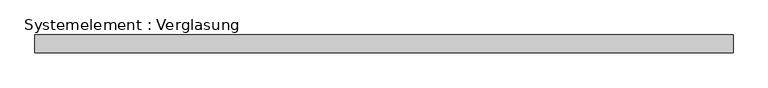
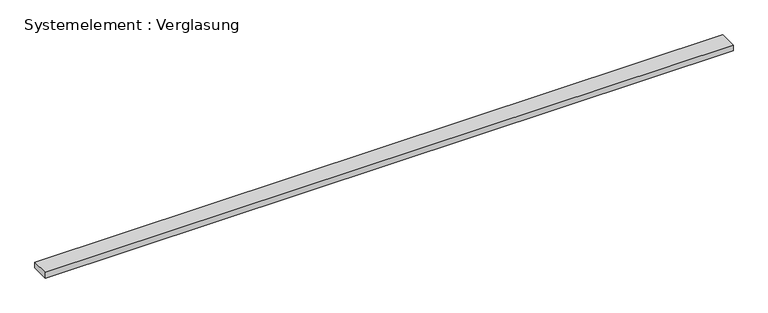
"""IFC4 building model written with IfcOpenShell, lengths in millimetres: plate geometry, Systemelement : Verglasung."""

from ifc_helpers import new_model, si_unit, origin, origin_with_axes, place, context, project, spatial, polyline, outline, extrude, source, transform, mapped, element, save


def systemelement_verglasung_1bc3a817(model_context):
    return source(origin(), model_context, "Body", "SweptSolid", [
        extrude(outline(polyline([(580.0000002, -15.0), (-580.0000002, -15.0), (-580.0000002, 15.0), (580.0000002, 15.0), (580.0000002, -15.0)])), origin_with_axes(), (0.0, 0.0, 1.0), 10.0),
    ])


if __name__ == "__main__":
    model = new_model("IFC4")
    model_context = context("Model", 3, world=origin())
    ifc_project = project(units=[si_unit("LENGTHUNIT", "METRE", prefix="MILLI")], contexts=[model_context])
    site = spatial("IfcSite", under=ifc_project)
    building = spatial("IfcBuilding", under=site)
    placement = place(None, origin())
    systemelement_verglasung_shape = systemelement_verglasung_1bc3a817(model_context)
    element("IfcPlate", 1, ObjectType="Systemelement : Verglasung", at=placement, inside=building, context=model_context, shape_type="MappedRepresentation", body=[
        mapped(systemelement_verglasung_shape, transform((0.0, 0.0, 0.0), x_axis=(1.0, 0.0, 0.0), y_axis=(0.0, 1.0, 0.0), z_axis=(0.0, 0.0, 1.0))),
    ])
    save(model, "model.ifc")

# Revit data of these elements
# Type "Systemelement : Verglasung"
#   Construction Type Id = "GSP4R"
#   Analytic Construction = "1/8 Zoll Pilkington-Verglasung einfach"
#   Visual Light Transmittance = 0.9
#   Solar Heat Gain Coefficient = 0.86
#   Heat Transfer Coefficient (U) = 6.7069 W/(m²·K)
# Element 1 (IfcPlate, "Systemelement : Verglasung")
#   Materials on its faces: "Glas"
# Materials
#   "Glas": class "Glas", colour RGB 0 0 255, transparency 0.75, Comments = "Render-Darstellung nicht aktualisiert ", Cost = 0
